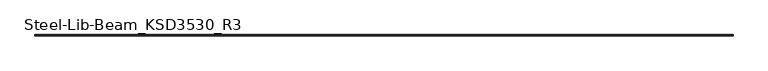
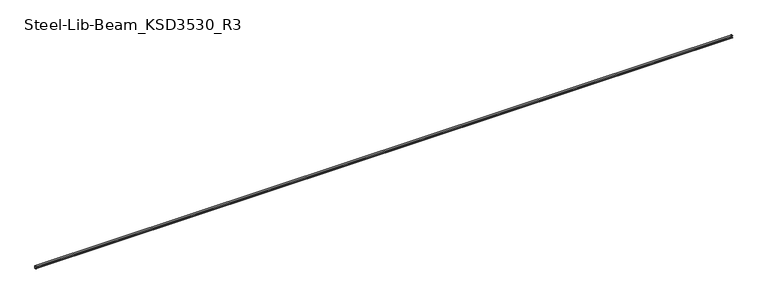
"""IFC4 building model written with IfcOpenShell, lengths in millimetres: beam geometry, Steel-Lib-Beam_KSD3530_R3 : BMS291_C-150×75x20x4.5."""

from ifc_helpers import new_model, si_unit, point, frame, frame_2d, origin, place, context, project, spatial, polyline, circle_curve, trimmed, segment, composite_curve, outline, extrude, source, transform, mapped, element, save


def steel_lib_beam_ksd3530_r3_22528ad0(model_context):
    return source(origin(), model_context, "Body", "SweptSolid", [
        extrude(outline(composite_curve([segment(trimmed(circle_curve(frame_2d((-41.0, 66.0)), 9.0), [point((-50.0, 66.0))], [point((-41.0, 75.0))], False, "CARTESIAN"), True, "CONTINUOUS"), segment(polyline([(-41.0, 75.0), (16.0, 75.0)]), True, "CONTINUOUS"), segment(trimmed(circle_curve(frame_2d((16.0, 66.0)), 9.0), [point((16.0, 75.0))], [point((25.0, 66.0))], False, "CARTESIAN"), True, "CONTINUOUS"), segment(polyline([(25.0, 66.0), (25.0, -66.0)]), True, "CONTINUOUS"), segment(trimmed(circle_curve(frame_2d((16.0, -66.0)), 9.0), [point((25.0, -66.0))], [point((16.0, -75.0))], False, "CARTESIAN"), True, "CONTINUOUS"), segment(polyline([(16.0, -75.0), (-41.0, -75.0)]), True, "CONTINUOUS"), segment(trimmed(circle_curve(frame_2d((-41.0, -66.0)), 9.0), [point((-41.0, -75.0))], [point((-50.0, -66.0))], False, "CARTESIAN"), True, "CONTINUOUS"), segment(polyline([(-50.0, -66.0), (-50.0, -55.0), (-45.5, -55.0), (-45.5, -66.0)]), True, "CONTINUOUS"), segment(trimmed(circle_curve(frame_2d((-41.0, -66.0)), 4.5), [point((-45.5, -66.0))], [point((-41.0, -70.5))], True, "CARTESIAN"), True, "CONTINUOUS"), segment(polyline([(-41.0, -70.5), (16.0, -70.5)]), True, "CONTINUOUS"), segment(trimmed(circle_curve(frame_2d((16.0, -66.0)), 4.5), [point((16.0, -70.5))], [point((20.5, -66.0))], True, "CARTESIAN"), True, "CONTINUOUS"), segment(polyline([(20.5, -66.0), (20.5, 66.0)]), True, "CONTINUOUS"), segment(trimmed(circle_curve(frame_2d((16.0, 66.0)), 4.5), [point((20.5, 66.0))], [point((16.0, 70.5))], True, "CARTESIAN"), True, "CONTINUOUS"), segment(polyline([(16.0, 70.5), (-41.0, 70.5)]), True, "CONTINUOUS"), segment(trimmed(circle_curve(frame_2d((-41.0, 66.0)), 4.5), [point((-41.0, 70.5))], [point((-45.5, 66.0))], True, "CARTESIAN"), True, "CONTINUOUS"), segment(polyline([(-45.5, 66.0), (-45.5, 55.0), (-50.0, 55.0), (-50.0, 66.0)]), True, "CONTINUOUS")], self_intersect=False)), frame((-20450.0, 0.0, 0.0), z_axis=(1.0, 0.0, 0.0), x_axis=(0.0, 1.0, 0.0)), (0.0, 0.0, 1.0), 40900.0),
    ])


if __name__ == "__main__":
    model = new_model("IFC4")
    model_context = context("Model", 3, world=origin())
    ifc_project = project(units=[si_unit("LENGTHUNIT", "METRE", prefix="MILLI")], contexts=[model_context])
    site = spatial("IfcSite", under=ifc_project)
    building = spatial("IfcBuilding", under=site)
    placement = place(None, origin())
    steel_lib_beam_ksd3530_r3_shape = steel_lib_beam_ksd3530_r3_22528ad0(model_context)
    element("IfcBeam", 1, ObjectType="Steel-Lib-Beam_KSD3530_R3 : BMS291_C-150×75x20x4.5", at=placement, inside=building, context=model_context, shape_type="MappedRepresentation", body=[
        mapped(steel_lib_beam_ksd3530_r3_shape, transform((0.0, 0.0, 0.0), x_axis=(1.0, 0.0, 0.0), y_axis=(0.0, 1.0, 0.0), z_axis=(0.0, 0.0, 1.0))),
    ])
    save(model, "model.ifc")

# Revit data of these elements
# Type "Steel-Lib-Beam_KSD3530_R3 : BMS291_C-150×75x20x4.5"
#   Keynote = "C-150×75x20x4.5"
#   SteelWeight = "Light"
#   x = 0.0250 m
#   t1 = 0.0090 m
#   t = 0.0045 m
#   Surface Area = 0.629834 m²/m
#   Section Area = 13.9688 cm²
#   Mass per Unit Length = 10.9655 kg/m
#   C = 0.0200 m
#   A = 0.0750 m
#   Length [instance default] = 1.5000 m
#   H = 0.1500 m
#   hec_material4 [instance default] = none
#   hec_material3 [instance default] = none
#   hec_material2 [instance default] = none
#   hec_material1 [instance default] = none
#   Structural Material [instance default] = Metal - Steel - Light Gauge
#   Assembly Code = ""
# Element 1 (IfcBeam, "Steel-Lib-Beam_KSD3530_R3 : BMS291_C-150×75x20x4.5")
#   Structural Material = none
# Materials
#   "Metal - Steel - Light Gauge": class "Metal", colour RGB 247 247 247, transparency 0
